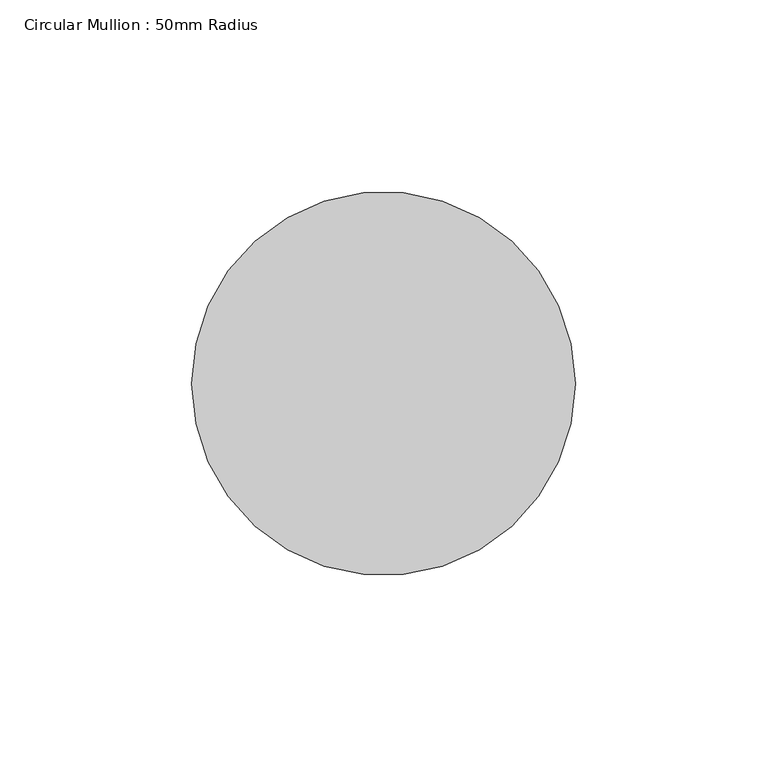
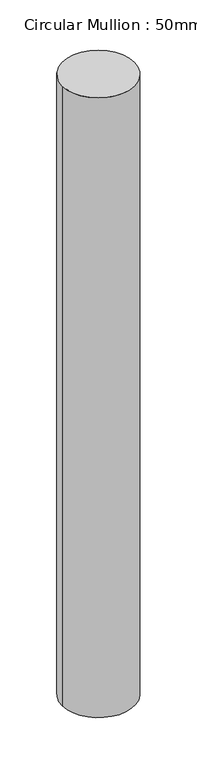
"""IFC4 building model written with IfcOpenShell, lengths in millimetres: member geometry, Circular Mullion : 50mm Radius."""

from ifc_helpers import new_model, si_unit, point, frame, origin, origin_2d, place, context, project, spatial, circle_curve, trimmed, segment, composite_curve, outline, extrude, source, transform, mapped, element, save


def circular_mullion_50mm_radius_55b9b966(model_context):
    return source(origin(), model_context, "Body", "SweptSolid", [
        extrude(outline(composite_curve([segment(trimmed(circle_curve(origin_2d(), 50.0), [point((50.0, 0.0))], [point((-50.0, 0.0))], False, "CARTESIAN"), True, "CONTINUOUS"), segment(trimmed(circle_curve(origin_2d(), 50.0), [point((-50.0, 0.0))], [point((50.0, 0.0))], False, "CARTESIAN"), True, "CONTINUOUS")], self_intersect=False)), frame((0.0, 0.0, -909.9059505), z_axis=(0.0, 0.0, 1.0), x_axis=(1.0, 0.0, 0.0)), (0.0, 0.0, 1.0), 909.9059505),
    ])


if __name__ == "__main__":
    model = new_model("IFC4")
    model_context = context("Model", 3, world=origin())
    ifc_project = project(units=[si_unit("LENGTHUNIT", "METRE", prefix="MILLI")], contexts=[model_context])
    site = spatial("IfcSite", under=ifc_project)
    building = spatial("IfcBuilding", under=site)
    placement = place(None, origin())
    circular_mullion_50mm_radius_shape = circular_mullion_50mm_radius_55b9b966(model_context)
    element("IfcMember", 1, ObjectType="Circular Mullion : 50mm Radius", at=placement, inside=building, context=model_context, shape_type="MappedRepresentation", body=[
        mapped(circular_mullion_50mm_radius_shape, transform((0.0, 0.0, 0.0), x_axis=(1.0, 0.0, 0.0), y_axis=(0.0, 1.0, 0.0), z_axis=(0.0, 0.0, 1.0))),
    ])
    save(model, "model.ifc")

# Revit data of these elements
# Type "Circular Mullion : 50mm Radius"
#   built-in parameter 1007350 = 0.164042 (stored number, unit not read)
# Element 1 (IfcMember, "Circular Mullion : 50mm Radius")
#   Materials on its faces: "Aluminium"
# Materials
#   "Aluminium": class "Metal", colour RGB 247 247 247, transparency 0, Description = "Aluminium 6061", Cost = 0
